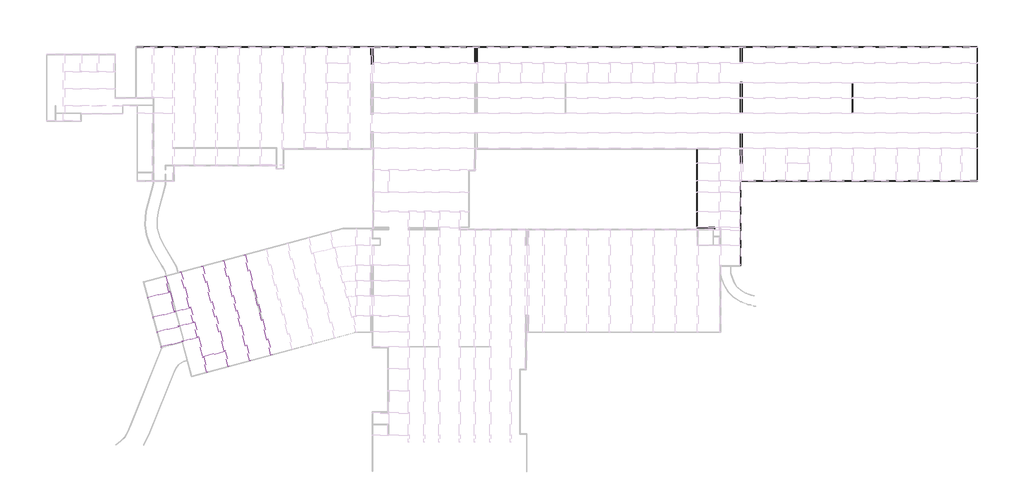
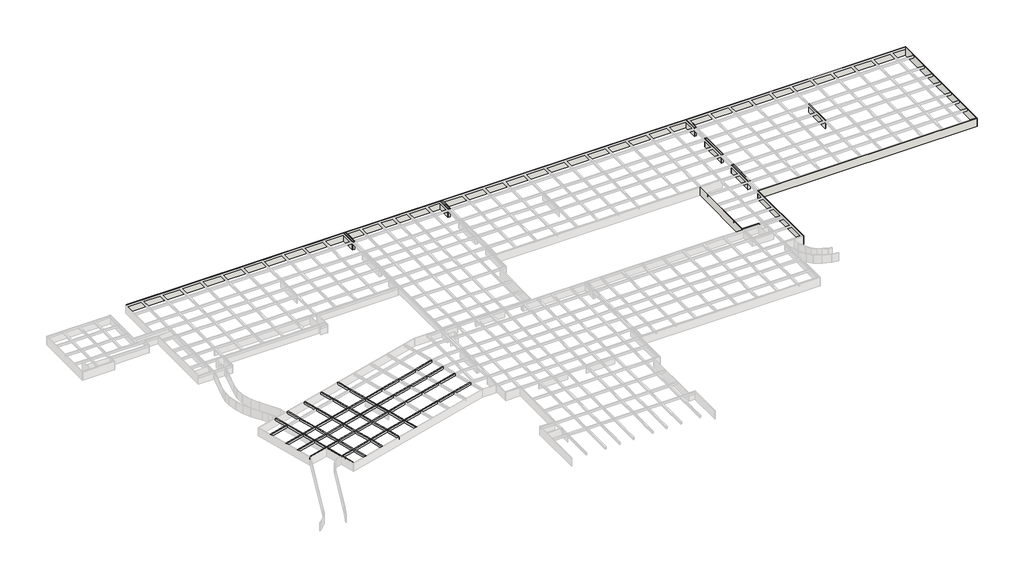
# One storey, part 3 of 14: 25 walls, 10 beams.
"""IFC4 building model written with IfcOpenShell, lengths in millimetres."""

from ifc_helpers import new_model, si_unit, frame, origin, origin_with_axes, place, context, project, spatial, polyline, outline, extrude, faceted_brep, element, save

model = new_model("IFC4")

# Units and contexts
model_context = context("Model", 3, world=origin())
ifc_project = project(units=[si_unit("LENGTHUNIT", "METRE", prefix="MILLI")], contexts=[model_context])

# Site, building, storey
site = spatial("IfcSite", under=ifc_project)
building = spatial("IfcBuilding", under=site)
storey = spatial("IfcBuildingStorey", under=building, Name="户型图", Elevation=0.0)

# Beams
placement = place(None, origin())
element("IfcBeam", 1, ObjectType="混凝土 - 矩形梁 : KL_beam", at=placement, inside=storey, context=model_context, shape_type="Brep", body=[
    faceted_brep([(-44965.652898, -232333.516161, 3300.0), (-45352.02323, -232437.0437735, 3300.0), (-45352.02323, -232437.0437735, 2500.0), (-44965.652898, -232333.516161, 2500.0), (-54495.3696285, -196768.1271004, 3300.0), (-54495.3696285, -196768.1271004, 2500.0), (-54881.7399605, -196871.6547129, 2500.0), (-54881.7399605, -196871.6547129, 3300.0), (-46371.3031308, -227087.5577736, 3300.0), (-46474.8307433, -226701.1874416, 3300.0), (-48238.8947773, -220117.6104614, 3300.0), (-48342.4223897, -219731.2401294, 3300.0), (-49654.0910999, -214836.0255798, 3300.0), (-49757.6187123, -214449.6552478, 3300.0), (-51037.0211351, -209674.8601288, 3300.0), (-51140.5487476, -209288.4897968, 3300.0), (-52926.4464378, -202623.4284974, 3300.0), (-53029.9740503, -202237.0581654, 3300.0), (-53416.344383, -202340.5857754, 3300.0), (-53312.8167705, -202726.9561074, 3300.0), (-51526.9190781, -209392.0174149, 3300.0), (-51423.3914656, -209778.3877469, 3300.0), (-50143.9890429, -214553.1828658, 3300.0), (-50040.4614304, -214939.5531978, 3300.0), (-48728.7927203, -219834.7677475, 3300.0), (-48625.2651078, -220221.1380795, 3300.0), (-46861.2010738, -226804.7150597, 3300.0), (-46757.6734613, -227191.0853917, 3300.0), (-53416.344383, -202340.5857754, 2500.0), (-53312.8167705, -202726.9561074, 2500.0), (-51526.9190781, -209392.0174149, 2500.0), (-51423.3914656, -209778.3877469, 2500.0), (-50143.9890429, -214553.1828658, 2500.0), (-50040.4614304, -214939.5531978, 2500.0), (-48728.7927203, -219834.7677475, 2500.0), (-48625.2651078, -220221.1380795, 2500.0), (-46861.2010738, -226804.7150597, 2500.0), (-46757.6734613, -227191.0853917, 2500.0), (-53029.9740503, -202237.0581654, 2500.0), (-52926.4464378, -202623.4284974, 2500.0), (-51140.5487476, -209288.4897968, 2500.0), (-51037.0211351, -209674.8601288, 2500.0), (-49757.6187123, -214449.6552478, 2500.0), (-49654.0910999, -214836.0255798, 2500.0), (-48342.4223897, -219731.2401294, 2500.0), (-48238.8947773, -220117.6104614, 2500.0), (-46474.8307433, -226701.1874416, 2500.0), (-46371.3031308, -227087.5577736, 2500.0)], [[[0, 1, 2, 3]], [[4, 5, 6, 7]], [[1, 0, 8, 9, 10, 11, 12, 13, 14, 15, 16, 17, 4, 7, 18, 19, 20, 21, 22, 23, 24, 25, 26, 27]], [[2, 1, 27, 26, 25, 24, 23, 22, 21, 20, 19, 18, 7, 6, 28, 29, 30, 31, 32, 33, 34, 35, 36, 37]], [[3, 2, 37, 36, 35, 34, 33, 32, 31, 30, 29, 28, 6, 5, 38, 39, 40, 41, 42, 43, 44, 45, 46, 47]], [[0, 3, 47, 46, 45, 44, 43, 42, 41, 40, 39, 38, 5, 4, 17, 16, 15, 14, 13, 12, 11, 10, 9, 8]]]),
])
element("IfcBeam", 2, ObjectType="混凝土 - 矩形梁 : KL_beam", at=placement, inside=storey, context=model_context, shape_type="Brep", body=[
    faceted_brep([(-47247.810521, -194958.9155951, 3300.0), (-46861.4401905, -194855.3879771, 3300.0), (-46861.4401905, -194855.3879771, 2500.0), (-47247.810521, -194958.9155951, 2500.0), (-37756.1396799, -230382.3134226, 3300.0), (-37756.1396799, -230382.3134226, 2500.0), (-37369.7693494, -230278.7858046, 2500.0), (-37369.7693494, -230278.7858046, 3300.0), (-45815.6063502, -200303.9743273, 3300.0), (-45712.0787322, -200690.3446578, 3300.0), (-43926.1809866, -207355.4057814, 3300.0), (-43822.6533686, -207741.7761119, 3300.0), (-42543.2508773, -212516.5712125, 3300.0), (-42439.7232593, -212902.941543, 3300.0), (-41128.054479, -217798.1560738, 3300.0), (-41024.5268609, -218184.5264043, 3300.0), (-39260.4627326, -224768.1033592, 3300.0), (-39156.9351145, -225154.4736897, 3300.0), (-38770.564784, -225050.9460717, 3300.0), (-38874.092402, -224664.5757412, 3300.0), (-40638.1565304, -218080.9987863, 3300.0), (-40741.6841484, -217694.6284558, 3300.0), (-42053.3529288, -212799.4139249, 3300.0), (-42156.8805468, -212413.0435944, 3300.0), (-43436.283038, -207638.2484938, 3300.0), (-43539.8106561, -207251.8781633, 3300.0), (-45325.7083995, -200586.8170478, 3300.0), (-45429.2360175, -200200.4467173, 3300.0), (-38770.564784, -225050.9460717, 2500.0), (-38874.092402, -224664.5757412, 2500.0), (-40638.1565304, -218080.9987863, 2500.0), (-40741.6841484, -217694.6284558, 2500.0), (-42053.3529288, -212799.4139249, 2500.0), (-42156.8805468, -212413.0435944, 2500.0), (-43436.283038, -207638.2484938, 2500.0), (-43539.8106561, -207251.8781633, 2500.0), (-45325.7083995, -200586.8170478, 2500.0), (-45429.2360175, -200200.4467173, 2500.0), (-39156.9351145, -225154.4736897, 2500.0), (-39260.4627326, -224768.1033592, 2500.0), (-41024.5268609, -218184.5264043, 2500.0), (-41128.054479, -217798.1560738, 2500.0), (-42439.7232593, -212902.941543, 2500.0), (-42543.2508773, -212516.5712125, 2500.0), (-43822.6533686, -207741.7761119, 2500.0), (-43926.1809866, -207355.4057814, 2500.0), (-45712.0787322, -200690.3446578, 2500.0), (-45815.6063502, -200303.9743273, 2500.0)], [[[0, 1, 2, 3]], [[4, 5, 6, 7]], [[1, 0, 8, 9, 10, 11, 12, 13, 14, 15, 16, 17, 4, 7, 18, 19, 20, 21, 22, 23, 24, 25, 26, 27]], [[2, 1, 27, 26, 25, 24, 23, 22, 21, 20, 19, 18, 7, 6, 28, 29, 30, 31, 32, 33, 34, 35, 36, 37]], [[3, 2, 37, 36, 35, 34, 33, 32, 31, 30, 29, 28, 6, 5, 38, 39, 40, 41, 42, 43, 44, 45, 46, 47]], [[0, 3, 47, 46, 45, 44, 43, 42, 41, 40, 39, 38, 5, 4, 17, 16, 15, 14, 13, 12, 11, 10, 9, 8]]]),
])
element("IfcBeam", 3, ObjectType="混凝土 - 矩形梁 : KL_beam", at=placement, inside=storey, context=model_context, shape_type="Brep", body=[
    faceted_brep([(-29827.2079849, -228304.2895391, 3300.0), (-30213.5783169, -228407.8171516, 3300.0), (-30213.5783169, -228407.8171516, 2500.0), (-29827.2079849, -228304.2895391, 2500.0), (-39323.7958794, -192862.5389847, 3300.0), (-39323.7958794, -192862.5389847, 2500.0), (-39710.1662114, -192966.0665972, 2500.0), (-39710.1662114, -192966.0665972, 3300.0), (-31239.6350842, -223033.0395404, 3300.0), (-31343.1626967, -222646.6692084, 3300.0), (-33107.2267306, -216063.0922282, 3300.0), (-33210.7543431, -215676.7218962, 3300.0), (-34522.4230532, -210781.5073465, 3300.0), (-34625.9506657, -210395.1370145, 3300.0), (-35905.3530884, -205620.3418956, 3300.0), (-36008.8807009, -205233.9715636, 3300.0), (-37794.7783067, -198568.9105793, 3300.0), (-37898.3059192, -198182.5402473, 3300.0), (-38284.6762519, -198286.0678573, 3300.0), (-38181.1486394, -198672.4381893, 3300.0), (-36395.2510314, -205337.4991816, 3300.0), (-36291.7234189, -205723.8695136, 3300.0), (-35012.3209962, -210498.6646326, 3300.0), (-34908.7933837, -210885.0349646, 3300.0), (-33597.1246736, -215780.2495142, 3300.0), (-33493.5970611, -216166.6198462, 3300.0), (-31729.5330272, -222750.1968264, 3300.0), (-31626.0054147, -223136.5671584, 3300.0), (-38284.6762519, -198286.0678573, 2500.0), (-38181.1486394, -198672.4381893, 2500.0), (-36395.2510314, -205337.4991816, 2500.0), (-36291.7234189, -205723.8695136, 2500.0), (-35012.3209962, -210498.6646326, 2500.0), (-34908.7933837, -210885.0349646, 2500.0), (-33597.1246736, -215780.2495142, 2500.0), (-33493.5970611, -216166.6198462, 2500.0), (-31729.5330272, -222750.1968264, 2500.0), (-31626.0054147, -223136.5671584, 2500.0), (-37898.3059192, -198182.5402473, 2500.0), (-37794.7783067, -198568.9105793, 2500.0), (-36008.8807009, -205233.9715636, 2500.0), (-35905.3530884, -205620.3418956, 2500.0), (-34625.9506657, -210395.1370145, 2500.0), (-34522.4230532, -210781.5073465, 2500.0), (-33210.7543431, -215676.7218962, 2500.0), (-33107.2267306, -216063.0922282, 2500.0), (-31343.1626967, -222646.6692084, 2500.0), (-31239.6350842, -223033.0395404, 2500.0)], [[[0, 1, 2, 3]], [[4, 5, 6, 7]], [[1, 0, 8, 9, 10, 11, 12, 13, 14, 15, 16, 17, 4, 7, 18, 19, 20, 21, 22, 23, 24, 25, 26, 27]], [[2, 1, 27, 26, 25, 24, 23, 22, 21, 20, 19, 18, 7, 6, 28, 29, 30, 31, 32, 33, 34, 35, 36, 37]], [[3, 2, 37, 36, 35, 34, 33, 32, 31, 30, 29, 28, 6, 5, 38, 39, 40, 41, 42, 43, 44, 45, 46, 47]], [[0, 3, 47, 46, 45, 44, 43, 42, 41, 40, 39, 38, 5, 4, 17, 16, 15, 14, 13, 12, 11, 10, 9, 8]]]),
])
element("IfcBeam", 4, ObjectType="混凝土 - 矩形梁 : KL_beam", at=placement, inside=storey, context=model_context, shape_type="Brep", body=[
    faceted_brep([(-32148.967433, -190913.2453078, 3300.0), (-31762.5971024, -190809.7176898, 3300.0), (-31762.5971024, -190809.7176898, 2500.0), (-32148.967433, -190913.2453078, 2500.0), (-22658.0730491, -226333.7453578, 3300.0), (-22658.0730491, -226333.7453578, 2500.0), (-22271.7027185, -226230.2177398, 2500.0), (-22271.7027185, -226230.2177398, 3300.0), (-30716.7763091, -196258.2553482, 3300.0), (-30613.2486911, -196644.6256787, 3300.0), (-28827.3510298, -203309.6864878, 3300.0), (-28723.8234117, -203696.0568183, 3300.0), (-27444.4209205, -208470.8519189, 3300.0), (-27340.8933025, -208857.2222494, 3300.0), (-26029.2245221, -213752.4367802, 3300.0), (-25925.6969041, -214138.8071108, 3300.0), (-24161.6327757, -220722.3840656, 3300.0), (-24058.1051577, -221108.7543962, 3300.0), (-23671.7348272, -221005.2267781, 3300.0), (-23775.2624452, -220618.8564476, 3300.0), (-25539.3265736, -214035.2794927, 3300.0), (-25642.8541916, -213648.9091622, 3300.0), (-26954.522972, -208753.6946314, 3300.0), (-27058.05059, -208367.3243008, 3300.0), (-28337.4530812, -203592.5292002, 3300.0), (-28440.9806993, -203206.1588697, 3300.0), (-30226.8783584, -196541.0980687, 3300.0), (-30330.4059764, -196154.7277382, 3300.0), (-23671.7348272, -221005.2267781, 2500.0), (-23775.2624452, -220618.8564476, 2500.0), (-25539.3265736, -214035.2794927, 2500.0), (-25642.8541916, -213648.9091622, 2500.0), (-26954.522972, -208753.6946314, 2500.0), (-27058.05059, -208367.3243008, 2500.0), (-28337.4530812, -203592.5292002, 2500.0), (-28440.9806993, -203206.1588697, 2500.0), (-30226.8783584, -196541.0980687, 2500.0), (-30330.4059764, -196154.7277382, 2500.0), (-24058.1051577, -221108.7543962, 2500.0), (-24161.6327757, -220722.3840656, 2500.0), (-25925.6969041, -214138.8071108, 2500.0), (-26029.2245221, -213752.4367802, 2500.0), (-27340.8933025, -208857.2222494, 2500.0), (-27444.4209205, -208470.8519189, 2500.0), (-28723.8234117, -203696.0568183, 2500.0), (-28827.3510298, -203309.6864878, 2500.0), (-30613.2486911, -196644.6256787, 2500.0), (-30716.7763091, -196258.2553482, 2500.0)], [[[0, 1, 2, 3]], [[4, 5, 6, 7]], [[1, 0, 8, 9, 10, 11, 12, 13, 14, 15, 16, 17, 4, 7, 18, 19, 20, 21, 22, 23, 24, 25, 26, 27]], [[2, 1, 27, 26, 25, 24, 23, 22, 21, 20, 19, 18, 7, 6, 28, 29, 30, 31, 32, 33, 34, 35, 36, 37]], [[3, 2, 37, 36, 35, 34, 33, 32, 31, 30, 29, 28, 6, 5, 38, 39, 40, 41, 42, 43, 44, 45, 46, 47]], [[0, 3, 47, 46, 45, 44, 43, 42, 41, 40, 39, 38, 5, 4, 17, 16, 15, 14, 13, 12, 11, 10, 9, 8]]]),
])
element("IfcBeam", 5, ObjectType="混凝土 - 矩形梁 : KL_beam", at=placement, inside=storey, context=model_context, shape_type="SweptSolid", body=[
    extrude(outline(polyline([(-66208.1826107, -206224.0134222), (-66313.6007329, -205838.1546145), (-58837.3326561, -203795.609192), (-58733.7322459, -204181.9646057), (-66208.1826107, -206224.0134222)])), frame((0.0, 0.0, 2500.0), z_axis=(0.0, 0.0, 1.0), x_axis=(1.0, 0.0, 0.0)), (0.0, 0.0, 1.0), 800.0),
])
element("IfcBeam", 6, ObjectType="混凝土 - 矩形梁 : KL_beam", at=placement, inside=storey, context=model_context, shape_type="Brep", body=[
    faceted_brep([(-64399.4506069, -212841.2018425, 3300.0), (-64399.4506069, -212841.2018425, 2500.0), (-64295.9229889, -213227.5721731, 2500.0), (-64295.9229889, -213227.5721731, 3300.0), (-51526.9190781, -209392.0174149, 3300.0), (-51423.3914656, -209778.3877469, 3300.0), (-51423.3914656, -209778.3877469, 2500.0), (-51526.9190781, -209392.0174149, 2500.0), (-56843.6193706, -211230.7334368, 3300.0), (-56457.2490334, -211127.205817, 3300.0), (-56560.8482958, -210740.8546835, 3300.0), (-56947.218633, -210844.3823033, 3300.0), (-56843.6193706, -211230.7334368, 2500.0), (-56457.2490334, -211127.205817, 2500.0), (-56947.218633, -210844.3823033, 2500.0), (-56560.8482958, -210740.8546835, 2500.0)], [[[0, 1, 2, 3]], [[4, 5, 6, 7]], [[0, 3, 8, 9, 5, 4, 10, 11]], [[3, 2, 12, 13, 6, 5, 9, 8]], [[2, 1, 14, 15, 7, 6, 13, 12]], [[1, 0, 11, 10, 4, 7, 15, 14]]]),
    faceted_brep([(-51140.5487476, -209288.4897968, 3300.0), (-51037.0211351, -209674.8601288, 3300.0), (-43822.6533686, -207741.7761119, 3300.0), (-43926.1809866, -207355.4057814, 3300.0), (-51037.0211351, -209674.8601288, 2500.0), (-43822.6533686, -207741.7761119, 2500.0), (-51140.5487476, -209288.4897968, 2500.0), (-43926.1809866, -207355.4057814, 2500.0)], [[[0, 1, 2, 3]], [[1, 4, 5, 2]], [[4, 6, 7, 5]], [[6, 0, 3, 7]], [[1, 0, 6, 4]], [[3, 2, 5, 7]]]),
    faceted_brep([(1279.8377522, -195242.4895673, 3300.0), (1383.3653703, -195628.8598978, 3300.0), (1383.3653703, -195628.8598978, 2500.0), (1279.8377522, -195242.4895673, 2500.0), (-5935.794677, -197175.9124495, 3300.0), (-5832.1954146, -197562.263583, 3300.0), (-5832.1954146, -197562.263583, 2500.0), (-5935.794677, -197175.9124495, 2500.0)], [[[0, 1, 2, 3]], [[1, 0, 4, 5]], [[2, 1, 5, 6]], [[3, 2, 6, 7]], [[0, 3, 7, 4]], [[5, 4, 7, 6]]]),
    faceted_brep([(-43436.283038, -207638.2484938, 3300.0), (-43539.8106561, -207251.8781633, 3300.0), (-43539.8106561, -207251.8781633, 2500.0), (-43436.283038, -207638.2484938, 2500.0), (-36395.2510314, -205337.4991816, 3300.0), (-36291.7234189, -205723.8695136, 3300.0), (-36291.7234189, -205723.8695136, 2500.0), (-36395.2510314, -205337.4991816, 2500.0)], [[[0, 1, 2, 3]], [[4, 5, 6, 7]], [[1, 0, 5, 4]], [[0, 3, 6, 5]], [[3, 2, 7, 6]], [[2, 1, 4, 7]]]),
    faceted_brep([(-36008.8807009, -205233.9715636, 3300.0), (-35905.3530884, -205620.3418956, 3300.0), (-28723.8234117, -203696.0568183, 3300.0), (-28827.3510298, -203309.6864878, 3300.0), (-35905.3530884, -205620.3418956, 2500.0), (-28723.8234117, -203696.0568183, 2500.0), (-36008.8807009, -205233.9715636, 2500.0), (-28827.3510298, -203309.6864878, 2500.0)], [[[0, 1, 2, 3]], [[1, 4, 5, 2]], [[4, 6, 7, 5]], [[6, 0, 3, 7]], [[1, 0, 6, 4]], [[3, 2, 5, 7]]]),
    faceted_brep([(-28337.4530812, -203592.5292002, 3300.0), (-28440.9806993, -203206.1588697, 3300.0), (-28440.9806993, -203206.1588697, 2500.0), (-28337.4530812, -203592.5292002, 2500.0), (-21391.9678165, -201317.3815604, 3300.0), (-21288.3685541, -201703.7326938, 3300.0), (-21288.3685541, -201703.7326938, 2500.0), (-21391.9678165, -201317.3815604, 2500.0)], [[[0, 1, 2, 3]], [[4, 5, 6, 7]], [[1, 0, 5, 4]], [[0, 3, 6, 5]], [[3, 2, 7, 6]], [[2, 1, 4, 7]]]),
    faceted_brep([(-21005.5974794, -201213.8539405, 3300.0), (-20901.9982169, -201600.205074, 3300.0), (-13710.1170819, -199673.1463318, 3300.0), (-13813.6447, -199286.7760013, 3300.0), (-20901.9982169, -201600.205074, 2500.0), (-13710.1170819, -199673.1463318, 2500.0), (-21005.5974794, -201213.8539405, 2500.0), (-13813.6447, -199286.7760013, 2500.0)], [[[0, 1, 2, 3]], [[1, 4, 5, 2]], [[4, 6, 7, 5]], [[6, 0, 3, 7]], [[1, 0, 6, 4]], [[3, 2, 5, 7]]]),
    faceted_brep([(-13323.7467514, -199569.6187138, 3300.0), (-13427.2743694, -199183.2483833, 3300.0), (-13427.2743694, -199183.2483833, 2500.0), (-13323.7467514, -199569.6187138, 2500.0), (-6322.1650141, -197279.4400694, 3300.0), (-6218.5657517, -197665.7912028, 3300.0), (-6218.5657517, -197665.7912028, 2500.0), (-6322.1650141, -197279.4400694, 2500.0)], [[[0, 1, 2, 3]], [[4, 5, 6, 7]], [[1, 0, 5, 4]], [[0, 3, 6, 5]], [[3, 2, 7, 6]], [[2, 1, 4, 7]]]),
])
element("IfcBeam", 7, ObjectType="混凝土 - 矩形梁 : KL_beam", at=placement, inside=storey, context=model_context, shape_type="Brep", body=[
    faceted_brep([(-62991.3282704, -217995.6170367, 3300.0), (-62991.3282704, -217995.6170367, 2500.0), (-62887.8006524, -218381.9873672, 2500.0), (-62887.8006524, -218381.9873672, 3300.0), (-50143.9890429, -214553.1828658, 3300.0), (-50040.4614304, -214939.5531978, 3300.0), (-50040.4614304, -214939.5531978, 2500.0), (-50143.9890429, -214553.1828658, 2500.0), (-55459.7322302, -216391.6424322, 3300.0), (-55073.361893, -216288.1148124, 3300.0), (-55176.9611554, -215901.7636789, 3300.0), (-55563.3314926, -216005.2912987, 3300.0), (-55459.7322302, -216391.6424322, 2500.0), (-55073.361893, -216288.1148124, 2500.0), (-55563.3314926, -216005.2912987, 2500.0), (-55176.9611554, -215901.7636789, 2500.0)], [[[0, 1, 2, 3]], [[4, 5, 6, 7]], [[0, 3, 8, 9, 5, 4, 10, 11]], [[3, 2, 12, 13, 6, 5, 9, 8]], [[2, 1, 14, 15, 7, 6, 13, 12]], [[1, 0, 11, 10, 4, 7, 15, 14]]]),
    faceted_brep([(-49757.6187123, -214449.6552478, 3300.0), (-49654.0910999, -214836.0255798, 3300.0), (-42439.7232593, -212902.941543, 3300.0), (-42543.2508773, -212516.5712125, 3300.0), (-49654.0910999, -214836.0255798, 2500.0), (-42439.7232593, -212902.941543, 2500.0), (-49757.6187123, -214449.6552478, 2500.0), (-42543.2508773, -212516.5712125, 2500.0)], [[[0, 1, 2, 3]], [[1, 4, 5, 2]], [[4, 6, 7, 5]], [[6, 0, 3, 7]], [[1, 0, 6, 4]], [[3, 2, 5, 7]]]),
    faceted_brep([(2662.7678615, -200403.6549984, 3300.0), (2766.2954795, -200790.0253289, 3300.0), (2766.2954795, -200790.0253289, 2500.0), (2662.7678615, -200403.6549984, 2500.0), (-4551.9075366, -202336.8214449, 3300.0), (-4448.3082742, -202723.1725784, 3300.0), (-4448.3082742, -202723.1725784, 2500.0), (-4551.9075366, -202336.8214449, 2500.0)], [[[0, 1, 2, 3]], [[1, 0, 4, 5]], [[2, 1, 5, 6]], [[3, 2, 6, 7]], [[0, 3, 7, 4]], [[5, 4, 7, 6]]]),
    faceted_brep([(-42053.3529288, -212799.4139249, 3300.0), (-42156.8805468, -212413.0435944, 3300.0), (-42156.8805468, -212413.0435944, 2500.0), (-42053.3529288, -212799.4139249, 2500.0), (-35012.3209962, -210498.6646326, 3300.0), (-34908.7933837, -210885.0349646, 3300.0), (-34908.7933837, -210885.0349646, 2500.0), (-35012.3209962, -210498.6646326, 2500.0)], [[[0, 1, 2, 3]], [[4, 5, 6, 7]], [[1, 0, 5, 4]], [[0, 3, 6, 5]], [[3, 2, 7, 6]], [[2, 1, 4, 7]]]),
    faceted_brep([(-34625.9506657, -210395.1370145, 3300.0), (-34522.4230532, -210781.5073465, 3300.0), (-27340.8933025, -208857.2222494, 3300.0), (-27444.4209205, -208470.8519189, 3300.0), (-34522.4230532, -210781.5073465, 2500.0), (-27340.8933025, -208857.2222494, 2500.0), (-34625.9506657, -210395.1370145, 2500.0), (-27444.4209205, -208470.8519189, 2500.0)], [[[0, 1, 2, 3]], [[1, 4, 5, 2]], [[4, 6, 7, 5]], [[6, 0, 3, 7]], [[1, 0, 6, 4]], [[3, 2, 5, 7]]]),
    faceted_brep([(-26954.522972, -208753.6946314, 3300.0), (-27058.05059, -208367.3243008, 3300.0), (-27058.05059, -208367.3243008, 2500.0), (-26954.522972, -208753.6946314, 2500.0), (-20008.0806761, -206478.2905558, 3300.0), (-19904.4814137, -206864.6416892, 3300.0), (-19904.4814137, -206864.6416892, 2500.0), (-20008.0806761, -206478.2905558, 2500.0)], [[[0, 1, 2, 3]], [[4, 5, 6, 7]], [[1, 0, 5, 4]], [[0, 3, 6, 5]], [[3, 2, 7, 6]], [[2, 1, 4, 7]]]),
    faceted_brep([(-19621.710339, -206374.7629359, 3300.0), (-19518.1110766, -206761.1140694, 3300.0), (-12327.1869726, -204834.3117629, 3300.0), (-12430.7145907, -204447.9414324, 3300.0), (-19518.1110766, -206761.1140694, 2500.0), (-12327.1869726, -204834.3117629, 2500.0), (-19621.710339, -206374.7629359, 2500.0), (-12430.7145907, -204447.9414324, 2500.0)], [[[0, 1, 2, 3]], [[1, 4, 5, 2]], [[4, 6, 7, 5]], [[6, 0, 3, 7]], [[1, 0, 6, 4]], [[3, 2, 5, 7]]]),
    faceted_brep([(-11940.8166421, -204730.7841449, 3300.0), (-12044.3442602, -204344.4138144, 3300.0), (-12044.3442602, -204344.4138144, 2500.0), (-11940.8166421, -204730.7841449, 2500.0), (-4938.2778738, -202440.3490648, 3300.0), (-4834.6786113, -202826.7001982, 3300.0), (-4834.6786113, -202826.7001982, 2500.0), (-4938.2778738, -202440.3490648, 2500.0)], [[[0, 1, 2, 3]], [[4, 5, 6, 7]], [[1, 0, 5, 4]], [[0, 3, 6, 5]], [[3, 2, 7, 6]], [[2, 1, 4, 7]]]),
])
element("IfcBeam", 8, ObjectType="混凝土 - 矩形梁 : KL_beam", at=placement, inside=storey, context=model_context, shape_type="Brep", body=[
    faceted_brep([(-61550.1618798, -223270.2432596, 3300.0), (-61550.1618798, -223270.2432596, 2500.0), (-61446.6342617, -223656.6135901, 2500.0), (-61446.6342617, -223656.6135901, 3300.0), (-48728.7927203, -219834.7677475, 3300.0), (-48625.2651078, -220221.1380795, 3300.0), (-48625.2651078, -220221.1380795, 2500.0), (-48728.7927203, -219834.7677475, 2500.0), (-54043.5564714, -221672.9648747, 3300.0), (-53657.1861343, -221569.4372549, 3300.0), (-53760.7853967, -221183.0861214, 3300.0), (-54147.1557338, -221286.6137413, 3300.0), (-54043.5564714, -221672.9648747, 2500.0), (-53657.1861343, -221569.4372549, 2500.0), (-54147.1557338, -221286.6137413, 2500.0), (-53760.7853967, -221183.0861214, 2500.0)], [[[0, 1, 2, 3]], [[4, 5, 6, 7]], [[0, 3, 8, 9, 5, 4, 10, 11]], [[3, 2, 12, 13, 6, 5, 9, 8]], [[2, 1, 14, 15, 7, 6, 13, 12]], [[1, 0, 11, 10, 4, 7, 15, 14]]]),
    faceted_brep([(-48342.4223897, -219731.2401294, 3300.0), (-48238.8947773, -220117.6104614, 3300.0), (-41024.5268609, -218184.5264043, 3300.0), (-41128.054479, -217798.1560738, 3300.0), (-48238.8947773, -220117.6104614, 2500.0), (-41024.5268609, -218184.5264043, 2500.0), (-48342.4223897, -219731.2401294, 2500.0), (-41128.054479, -217798.1560738, 2500.0)], [[[0, 1, 2, 3]], [[1, 4, 5, 2]], [[4, 6, 7, 5]], [[6, 0, 3, 7]], [[1, 0, 6, 4]], [[3, 2, 5, 7]]]),
    faceted_brep([(4077.9642599, -205685.2398597, 3300.0), (4181.4918779, -206071.6101903, 3300.0), (4181.4918779, -206071.6101903, 2500.0), (4077.9642599, -205685.2398597, 2500.0), (-3135.7317778, -207618.1438875, 3300.0), (-3032.1325154, -208004.4950209, 3300.0), (-3032.1325154, -208004.4950209, 2500.0), (-3135.7317778, -207618.1438875, 2500.0)], [[[0, 1, 2, 3]], [[1, 0, 4, 5]], [[2, 1, 5, 6]], [[3, 2, 6, 7]], [[0, 3, 7, 4]], [[5, 4, 7, 6]]]),
    faceted_brep([(-40638.1565304, -218080.9987863, 3300.0), (-40741.6841484, -217694.6284558, 3300.0), (-40741.6841484, -217694.6284558, 2500.0), (-40638.1565304, -218080.9987863, 2500.0), (-33597.1246736, -215780.2495142, 3300.0), (-33493.5970611, -216166.6198462, 3300.0), (-33493.5970611, -216166.6198462, 2500.0), (-33597.1246736, -215780.2495142, 2500.0)], [[[0, 1, 2, 3]], [[4, 5, 6, 7]], [[1, 0, 5, 4]], [[0, 3, 6, 5]], [[3, 2, 7, 6]], [[2, 1, 4, 7]]]),
    faceted_brep([(-33210.7543431, -215676.7218962, 3300.0), (-33107.2267306, -216063.0922282, 3300.0), (-25925.6969041, -214138.8071108, 3300.0), (-26029.2245221, -213752.4367802, 3300.0), (-33107.2267306, -216063.0922282, 2500.0), (-25925.6969041, -214138.8071108, 2500.0), (-33210.7543431, -215676.7218962, 2500.0), (-26029.2245221, -213752.4367802, 2500.0)], [[[0, 1, 2, 3]], [[1, 4, 5, 2]], [[4, 6, 7, 5]], [[6, 0, 3, 7]], [[1, 0, 6, 4]], [[3, 2, 5, 7]]]),
    faceted_brep([(-25539.3265736, -214035.2794927, 3300.0), (-25642.8541916, -213648.9091622, 3300.0), (-25642.8541916, -213648.9091622, 2500.0), (-25539.3265736, -214035.2794927, 2500.0), (-18591.9049174, -211759.6129983, 3300.0), (-18488.305655, -212145.9641318, 3300.0), (-18488.305655, -212145.9641318, 2500.0), (-18591.9049174, -211759.6129983, 2500.0)], [[[0, 1, 2, 3]], [[4, 5, 6, 7]], [[1, 0, 5, 4]], [[0, 3, 6, 5]], [[3, 2, 7, 6]], [[2, 1, 4, 7]]]),
    faceted_brep([(-18205.5345802, -211656.0853785, 3300.0), (-18101.9353178, -212042.4365119, 3300.0), (-10911.9905743, -210115.8966243, 3300.0), (-11015.5181923, -209729.5262938, 3300.0), (-18101.9353178, -212042.4365119, 2500.0), (-10911.9905743, -210115.8966243, 2500.0), (-18205.5345802, -211656.0853785, 2500.0), (-11015.5181923, -209729.5262938, 2500.0)], [[[0, 1, 2, 3]], [[1, 4, 5, 2]], [[4, 6, 7, 5]], [[6, 0, 3, 7]], [[1, 0, 6, 4]], [[3, 2, 5, 7]]]),
    faceted_brep([(-10525.6202438, -210012.3690062, 3300.0), (-10629.1478618, -209625.9986757, 3300.0), (-10629.1478618, -209625.9986757, 2500.0), (-10525.6202438, -210012.3690062, 2500.0), (-3522.102115, -207721.6715073, 3300.0), (-3418.5028526, -208108.0226408, 3300.0), (-3418.5028526, -208108.0226408, 2500.0), (-3522.102115, -207721.6715073, 2500.0)], [[[0, 1, 2, 3]], [[4, 5, 6, 7]], [[1, 0, 5, 4]], [[0, 3, 6, 5]], [[3, 2, 7, 6]], [[2, 1, 4, 7]]]),
])
element("IfcBeam", 9, ObjectType="混凝土 - 矩形梁 : KL_beam", at=placement, inside=storey, context=model_context, shape_type="SweptSolid", body=[
    extrude(outline(polyline([(5945.5560063, -212655.1871451), (6049.0836243, -213041.5574756), (-1163.2483368, -214974.0960002), (-1266.8475992, -214587.7448667), (5945.5560063, -212655.1871451)])), frame((0.0, 0.0, 2500.0), z_axis=(0.0, 0.0, 1.0), x_axis=(1.0, 0.0, 0.0)), (0.0, 0.0, 1.0), 800.0),
    extrude(outline(polyline([(-46861.2010738, -226804.7150597), (-46757.6734613, -227191.0853917), (-51788.3019556, -228539.0382341), (-51891.9012181, -228152.6871007), (-46861.2010738, -226804.7150597)])), frame((0.0, 0.0, 2500.0), z_axis=(0.0, 0.0, 1.0), x_axis=(1.0, 0.0, 0.0)), (0.0, 0.0, 1.0), 800.0),
    extrude(outline(polyline([(-46371.3031308, -227087.5577736), (-46474.8307433, -226701.1874416), (-39260.4627326, -224768.1033592), (-39156.9351145, -225154.4736897), (-46371.3031308, -227087.5577736)])), frame((0.0, 0.0, 2500.0), z_axis=(0.0, 0.0, 1.0), x_axis=(1.0, 0.0, 0.0)), (0.0, 0.0, 1.0), 800.0),
    extrude(outline(polyline([(-31626.0054147, -223136.5671584), (-38770.564784, -225050.9460717), (-38874.092402, -224664.5757412), (-31729.5330272, -222750.1968264), (-31626.0054147, -223136.5671584)])), frame((0.0, 0.0, 2500.0), z_axis=(0.0, 0.0, 1.0), x_axis=(1.0, 0.0, 0.0)), (0.0, 0.0, 1.0), 800.0),
    extrude(outline(polyline([(-24058.1051577, -221108.7543962), (-31239.6350842, -223033.0395404), (-31343.1626967, -222646.6692084), (-24161.6327757, -220722.3840656), (-24058.1051577, -221108.7543962)])), frame((0.0, 0.0, 2500.0), z_axis=(0.0, 0.0, 1.0), x_axis=(1.0, 0.0, 0.0)), (0.0, 0.0, 1.0), 800.0),
    extrude(outline(polyline([(-16619.4214764, -219115.565111), (-23671.7348272, -221005.2267781), (-23775.2624452, -220618.8564476), (-16723.0207388, -218729.2139775), (-16619.4214764, -219115.565111)])), frame((0.0, 0.0, 2500.0), z_axis=(0.0, 0.0, 1.0), x_axis=(1.0, 0.0, 0.0)), (0.0, 0.0, 1.0), 800.0),
    extrude(outline(polyline([(-9044.3988279, -217085.8439097), (-16233.0511392, -219012.0374912), (-16336.6504016, -218625.6863577), (-9147.9264459, -216699.4735792), (-9044.3988279, -217085.8439097)])), frame((0.0, 0.0, 2500.0), z_axis=(0.0, 0.0, 1.0), x_axis=(1.0, 0.0, 0.0)), (0.0, 0.0, 1.0), 800.0),
    extrude(outline(polyline([(-1549.618674, -215077.62362), (-8658.0284974, -216982.3162916), (-8761.5561154, -216595.9459611), (-1653.2179364, -214691.2724865), (-1549.618674, -215077.62362)])), frame((0.0, 0.0, 2500.0), z_axis=(0.0, 0.0, 1.0), x_axis=(1.0, 0.0, 0.0)), (0.0, 0.0, 1.0), 800.0),
])
element("IfcBeam", 10, ObjectType="混凝土 - 矩形梁 : KL_beam", at=placement, inside=storey, context=model_context, shape_type="Brep", body=[
    faceted_brep([(-50406.0295376, -233693.9254706, 3300.0), (-50792.3806644, -233797.5247312, 3300.0), (-50792.3806644, -233797.5247312, 2500.0), (-50406.0295376, -233693.9254706, 2500.0), (-51788.3019556, -228539.0382341, 3300.0), (-51891.9012181, -228152.6871007, 3300.0), (-53657.1861343, -221569.4372549, 3300.0), (-54043.5564714, -221672.9648747, 3300.0), (-54043.5564714, -221672.9648747, 2500.0), (-53657.1861343, -221569.4372549, 2500.0), (-51891.9012181, -228152.6871007, 2500.0), (-51788.3019556, -228539.0382341, 2500.0)], [[[0, 1, 2, 3]], [[1, 0, 4, 5, 6, 7]], [[2, 1, 7, 8]], [[3, 2, 8, 9, 10, 11]], [[0, 3, 11, 10, 9, 6, 5, 4]], [[7, 6, 9, 8]]]),
    faceted_brep([(-59881.2179144, -198358.2514113, 3300.0), (-59881.2179144, -198358.2514113, 2500.0), (-60267.5690413, -198461.8506719, 2500.0), (-60267.5690413, -198461.8506719, 3300.0), (-56560.8482958, -210740.8546835, 3300.0), (-56947.218633, -210844.3823033, 3300.0), (-56947.218633, -210844.3823033, 2500.0), (-56560.8482958, -210740.8546835, 2500.0), (-58837.3326561, -203795.609192, 3300.0), (-58733.7322459, -204181.9646057, 3300.0), (-58347.9820093, -204076.1244544, 3300.0), (-58451.5812717, -203689.773321, 3300.0), (-58837.3326561, -203795.609192, 2500.0), (-58733.7322459, -204181.9646057, 2500.0), (-58451.5812717, -203689.773321, 2500.0), (-58347.9820093, -204076.1244544, 2500.0)], [[[0, 1, 2, 3]], [[4, 5, 6, 7]], [[0, 3, 8, 9, 5, 4, 10, 11]], [[3, 2, 12, 13, 6, 5, 9, 8]], [[2, 1, 14, 15, 7, 6, 13, 12]], [[1, 0, 11, 10, 4, 7, 15, 14]]]),
    faceted_brep([(-56843.6193706, -211230.7334368, 3300.0), (-56457.2490334, -211127.205817, 3300.0), (-56457.2490334, -211127.205817, 2500.0), (-56843.6193706, -211230.7334368, 2500.0), (-55176.9611554, -215901.7636789, 3300.0), (-55563.3314926, -216005.2912987, 3300.0), (-55563.3314926, -216005.2912987, 2500.0), (-55176.9611554, -215901.7636789, 2500.0)], [[[0, 1, 2, 3]], [[4, 5, 6, 7]], [[1, 0, 5, 4]], [[0, 3, 6, 5]], [[3, 2, 7, 6]], [[2, 1, 4, 7]]]),
    faceted_brep([(-55459.7322302, -216391.6424322, 3300.0), (-55073.361893, -216288.1148124, 3300.0), (-55073.361893, -216288.1148124, 2500.0), (-55459.7322302, -216391.6424322, 2500.0), (-53760.7853967, -221183.0861214, 3300.0), (-54147.1557338, -221286.6137413, 3300.0), (-54147.1557338, -221286.6137413, 2500.0), (-53760.7853967, -221183.0861214, 2500.0)], [[[0, 1, 2, 3]], [[4, 5, 6, 7]], [[1, 0, 5, 4]], [[0, 3, 6, 5]], [[3, 2, 7, 6]], [[2, 1, 4, 7]]]),
])

# Walls
element("IfcWall", 11, ObjectType="所有墙体", at=placement, inside=storey, context=model_context, shape_type="Brep", body=[
    faceted_brep([(-70312.7050956, -117418.950757, 0.0), (12717.2949044, -117418.950757, 0.0), (12837.2949044, -117418.950757, 0.0), (13417.2949044, -117418.950757, 0.0), (13537.2949044, -117418.950757, 0.0), (49516.5330009, -117418.950757, 0.0), (49636.5330009, -117418.950757, 0.0), (50217.2949044, -117418.950757, 0.0), (50337.2949044, -117418.950757, 0.0), (143317.2949044, -117418.950757, 0.0), (143437.2949044, -117418.950757, 0.0), (144017.2949044, -117418.950757, 0.0), (144137.2949044, -117418.950757, 0.0), (227167.2949044, -117418.950757, 0.0), (227287.2949044, -117418.950757, 0.0), (227287.2949044, -117418.950757, 3300.0), (227167.2949044, -117418.950757, 3300.0), (144137.2949044, -117418.950757, 3300.0), (144017.2949044, -117418.950757, 3300.0), (143437.2949044, -117418.950757, 3300.0), (143317.2949044, -117418.950757, 3300.0), (50337.2949044, -117418.950757, 3300.0), (50217.2949044, -117418.950757, 3300.0), (49636.5330009, -117418.950757, 3300.0), (49516.5330009, -117418.950757, 3300.0), (13537.2949044, -117418.950757, 3300.0), (13417.2949044, -117418.950757, 3300.0), (12837.2949044, -117418.950757, 3300.0), (12717.2949044, -117418.950757, 3300.0), (-70312.7050956, -117418.950757, 3300.0), (-70312.7050956, -117298.950757, 0.0), (-70312.7050956, -117298.950757, 3300.0), (227287.2949044, -117298.950757, 3300.0), (227287.2949044, -117298.950757, 0.0)], [[[0, 1, 2, 3, 4, 5, 6, 7, 8, 9, 10, 11, 12, 13, 14, 15, 16, 17, 18, 19, 20, 21, 22, 23, 24, 25, 26, 27, 28, 29]], [[30, 31, 32, 33]], [[14, 13, 12, 11, 10, 9, 8, 7, 6, 5, 4, 3, 2, 1, 0, 30, 33]], [[29, 28, 27, 26, 25, 24, 23, 22, 21, 20, 19, 18, 17, 16, 15, 32, 31]], [[0, 29, 31, 30]], [[15, 14, 33, 32]]]),
])
element("IfcWall", 12, ObjectType="所有墙体", at=placement, inside=storey, context=model_context, shape_type="Brep", body=[
    faceted_brep([(227167.2949044, -117418.950757, 0.0), (227167.2949044, -164696.0449275, 0.0), (227167.2949044, -164816.0449275, 0.0), (227167.2949044, -164816.0449275, 3300.0), (227167.2949044, -164696.0449275, 3300.0), (227167.2949044, -117418.950757, 3300.0), (227287.2949044, -117418.950757, 0.0), (227287.2949044, -117418.950757, 3300.0), (227287.2949044, -164816.0449275, 3300.0), (227287.2949044, -164816.0449275, 0.0)], [[[0, 1, 2, 3, 4, 5]], [[6, 7, 8, 9]], [[2, 1, 0, 6, 9]], [[5, 4, 3, 8, 7]], [[0, 5, 7, 6]], [[3, 2, 9, 8]]]),
])
element("IfcWall", 13, ObjectType="所有墙体", at=placement, inside=storey, context=model_context, shape_type="Brep", body=[
    faceted_brep([(227167.2949044, -164696.0449275, 0.0), (143467.2949044, -164696.0449275, 0.0), (143467.2949044, -164696.0449275, 3300.0), (227167.2949044, -164696.0449275, 3300.0), (227167.2949044, -164816.0449275, 0.0), (227167.2949044, -164816.0449275, 3300.0), (143587.2949044, -164816.0449275, 3300.0), (143467.2949044, -164816.0449275, 3300.0), (143467.2949044, -164816.0449275, 0.0), (143587.2949044, -164816.0449275, 0.0)], [[[0, 1, 2, 3]], [[4, 5, 6, 7, 8, 9]], [[1, 0, 4, 9, 8]], [[3, 2, 7, 6, 5]], [[0, 3, 5, 4]], [[2, 1, 8, 7]]]),
])
element("IfcWall", 14, ObjectType="所有墙体", at=placement, inside=storey, context=model_context, shape_type="Brep", body=[
    faceted_brep([(143467.2949044, -164816.0449275, 0.0), (143467.2949044, -194796.0449275, 0.0), (143467.2949044, -194916.0449275, 0.0), (143467.2949044, -194916.0449275, 3300.0), (143467.2949044, -194796.0449275, 3300.0), (143467.2949044, -164816.0449275, 3300.0), (143587.2949044, -164816.0449275, 0.0), (143587.2949044, -164816.0449275, 3300.0), (143587.2949044, -194916.0449275, 3300.0), (143587.2949044, -194916.0449275, 0.0)], [[[0, 1, 2, 3, 4, 5]], [[6, 7, 8, 9]], [[2, 1, 0, 6, 9]], [[5, 4, 3, 8, 7]], [[0, 5, 7, 6]], [[3, 2, 9, 8]]]),
])
element("IfcWall", 15, ObjectType="所有墙体", at=placement, inside=storey, context=model_context, shape_type="Brep", body=[
    faceted_brep([(134428.3552546, -181848.950757, 0.0), (134428.3552546, -181148.950757, 0.0), (134428.3552546, -181148.950757, 3300.0), (134428.3552546, -181848.950757, 3300.0), (134308.3552546, -181848.950757, 0.0), (134308.3552546, -181848.950757, 3300.0), (134308.3552546, -181268.950757, 3300.0), (134308.3552546, -181148.950757, 3300.0), (134308.3552546, -181148.950757, 0.0), (134308.3552546, -181268.950757, 0.0)], [[[0, 1, 2, 3]], [[4, 5, 6, 7, 8, 9]], [[1, 0, 4, 9, 8]], [[3, 2, 7, 6, 5]], [[0, 3, 5, 4]], [[2, 1, 8, 7]]]),
])
element("IfcWall", 16, ObjectType="所有墙体", at=placement, inside=storey, context=model_context, shape_type="Brep", body=[
    faceted_brep([(134308.3552546, -181148.950757, 0.0), (128087.2949044, -181148.950757, 0.0), (127967.2949044, -181148.950757, 0.0), (127967.2949044, -181148.950757, 3300.0), (128087.2949044, -181148.950757, 3300.0), (134308.3552546, -181148.950757, 3300.0), (134308.3552546, -181268.950757, 0.0), (134308.3552546, -181268.950757, 3300.0), (127967.2949044, -181268.950757, 3300.0), (127967.2949044, -181268.950757, 0.0)], [[[0, 1, 2, 3, 4, 5]], [[6, 7, 8, 9]], [[2, 1, 0, 6, 9]], [[5, 4, 3, 8, 7]], [[0, 5, 7, 6]], [[3, 2, 9, 8]]]),
])
element("IfcWall", 17, ObjectType="所有墙体", at=placement, inside=storey, context=model_context, shape_type="SweptSolid", body=[
    extrude(outline(polyline([(128087.2949044, -153418.950757), (128087.2949044, -181148.950757), (127967.2949044, -181148.950757), (127967.2949044, -153418.950757), (128087.2949044, -153418.950757)])), origin_with_axes(), (0.0, 0.0, 1.0), 3300.0),
])
element("IfcWall", 18, ObjectType="所有墙体", at=placement, inside=storey, context=model_context, shape_type="Brep", body=[
    faceted_brep([(143317.2949044, -158518.950757, 0.0), (144137.2949044, -158518.950757, 0.0), (144137.2949044, -158518.950757, 3300.0), (143317.2949044, -158518.950757, 3300.0), (143317.2949044, -158398.950757, 0.0), (143317.2949044, -158398.950757, 3300.0), (143437.2949044, -158398.950757, 3300.0), (144017.2949044, -158398.950757, 3300.0), (144137.2949044, -158398.950757, 3300.0), (144137.2949044, -158398.950757, 0.0), (144017.2949044, -158398.950757, 0.0), (143437.2949044, -158398.950757, 0.0)], [[[0, 1, 2, 3]], [[4, 5, 6, 7, 8, 9, 10, 11]], [[1, 0, 4, 11, 10, 9]], [[3, 2, 8, 7, 6, 5]], [[2, 1, 9, 8]], [[0, 3, 5, 4]]]),
])
element("IfcWall", 19, ObjectType="所有墙体", at=placement, inside=storey, context=model_context, shape_type="Brep", body=[
    faceted_brep([(144137.2949044, -158398.950757, 0.0), (144137.2949044, -147598.950757, 0.0), (144137.2949044, -147598.950757, 3300.0), (144137.2949044, -158398.950757, 3300.0), (144017.2949044, -158398.950757, 0.0), (144017.2949044, -158398.950757, 3300.0), (144017.2949044, -147718.950757, 3300.0), (144017.2949044, -147598.950757, 3300.0), (144017.2949044, -147598.950757, 0.0), (144017.2949044, -147718.950757, 0.0)], [[[0, 1, 2, 3]], [[4, 5, 6, 7, 8, 9]], [[1, 0, 4, 9, 8]], [[3, 2, 7, 6, 5]], [[0, 3, 5, 4]], [[2, 1, 8, 7]]]),
])
element("IfcWall", 20, ObjectType="所有墙体", at=placement, inside=storey, context=model_context, shape_type="Brep", body=[
    faceted_brep([(144017.2949044, -147598.950757, 0.0), (143317.2949044, -147598.950757, 0.0), (143317.2949044, -147598.950757, 3300.0), (144017.2949044, -147598.950757, 3300.0), (144017.2949044, -147718.950757, 0.0), (144017.2949044, -147718.950757, 3300.0), (143437.2949044, -147718.950757, 3300.0), (143317.2949044, -147718.950757, 3300.0), (143317.2949044, -147718.950757, 0.0), (143437.2949044, -147718.950757, 0.0)], [[[0, 1, 2, 3]], [[4, 5, 6, 7, 8, 9]], [[1, 0, 4, 9, 8]], [[3, 2, 7, 6, 5]], [[0, 3, 5, 4]], [[2, 1, 8, 7]]]),
])
element("IfcWall", 21, ObjectType="所有墙体", at=placement, inside=storey, context=model_context, shape_type="SweptSolid", body=[
    extrude(outline(polyline([(143317.2949044, -158398.950757), (143317.2949044, -147718.950757), (143437.2949044, -147718.950757), (143437.2949044, -158398.950757), (143317.2949044, -158398.950757)])), origin_with_axes(), (0.0, 0.0, 1.0), 3300.0),
])
element("IfcWall", 22, ObjectType="所有墙体", at=placement, inside=storey, context=model_context, shape_type="Brep", body=[
    faceted_brep([(143317.2949044, -140845.610884, 0.0), (144137.2949044, -140845.610884, 0.0), (144137.2949044, -140845.610884, 3300.0), (143317.2949044, -140845.610884, 3300.0), (143317.2949044, -140725.610884, 0.0), (143317.2949044, -140725.610884, 3300.0), (143437.2949044, -140725.610884, 3300.0), (144017.2949044, -140725.610884, 3300.0), (144137.2949044, -140725.610884, 3300.0), (144137.2949044, -140725.610884, 0.0), (144017.2949044, -140725.610884, 0.0), (143437.2949044, -140725.610884, 0.0)], [[[0, 1, 2, 3]], [[4, 5, 6, 7, 8, 9, 10, 11]], [[1, 0, 4, 11, 10, 9]], [[3, 2, 8, 7, 6, 5]], [[2, 1, 9, 8]], [[0, 3, 5, 4]]]),
])
element("IfcWall", 23, ObjectType="所有墙体", at=placement, inside=storey, context=model_context, shape_type="Brep", body=[
    faceted_brep([(144137.2949044, -140725.610884, 0.0), (144137.2949044, -129856.524025, 0.0), (144137.2949044, -129856.524025, 3300.0), (144137.2949044, -140725.610884, 3300.0), (144017.2949044, -140725.610884, 0.0), (144017.2949044, -140725.610884, 3300.0), (144017.2949044, -129976.524025, 3300.0), (144017.2949044, -129856.524025, 3300.0), (144017.2949044, -129856.524025, 0.0), (144017.2949044, -129976.524025, 0.0)], [[[0, 1, 2, 3]], [[4, 5, 6, 7, 8, 9]], [[1, 0, 4, 9, 8]], [[3, 2, 7, 6, 5]], [[0, 3, 5, 4]], [[2, 1, 8, 7]]]),
])
element("IfcWall", 24, ObjectType="所有墙体", at=placement, inside=storey, context=model_context, shape_type="Brep", body=[
    faceted_brep([(144017.2949044, -129856.524025, 0.0), (143317.2949044, -129856.524025, 0.0), (143317.2949044, -129856.524025, 3300.0), (144017.2949044, -129856.524025, 3300.0), (144017.2949044, -129976.524025, 0.0), (144017.2949044, -129976.524025, 3300.0), (143437.2949044, -129976.524025, 3300.0), (143317.2949044, -129976.524025, 3300.0), (143317.2949044, -129976.524025, 0.0), (143437.2949044, -129976.524025, 0.0)], [[[0, 1, 2, 3]], [[4, 5, 6, 7, 8, 9]], [[1, 0, 4, 9, 8]], [[3, 2, 7, 6, 5]], [[0, 3, 5, 4]], [[2, 1, 8, 7]]]),
])
element("IfcWall", 25, ObjectType="所有墙体", at=placement, inside=storey, context=model_context, shape_type="SweptSolid", body=[
    extrude(outline(polyline([(143317.2949044, -140725.610884), (143317.2949044, -129976.524025), (143437.2949044, -129976.524025), (143437.2949044, -140725.610884), (143317.2949044, -140725.610884)])), origin_with_axes(), (0.0, 0.0, 1.0), 3300.0),
])
element("IfcWall", 26, ObjectType="所有墙体", at=placement, inside=storey, context=model_context, shape_type="Brep", body=[
    faceted_brep([(143317.2949044, -117418.950757, 0.0), (143317.2949044, -122999.5798504, 0.0), (143317.2949044, -122999.5798504, 3300.0), (143317.2949044, -117418.950757, 3300.0), (143437.2949044, -117418.950757, 0.0), (143437.2949044, -117418.950757, 3300.0), (143437.2949044, -122879.5798504, 3300.0), (143437.2949044, -122999.5798504, 3300.0), (143437.2949044, -122999.5798504, 0.0), (143437.2949044, -122879.5798504, 0.0)], [[[0, 1, 2, 3]], [[4, 5, 6, 7, 8, 9]], [[1, 0, 4, 9, 8]], [[3, 2, 7, 6, 5]], [[0, 3, 5, 4]], [[2, 1, 8, 7]]]),
])
element("IfcWall", 27, ObjectType="所有墙体", at=placement, inside=storey, context=model_context, shape_type="Brep", body=[
    faceted_brep([(143437.2949044, -122999.5798504, 0.0), (144137.2949044, -122999.5798504, 0.0), (144137.2949044, -122999.5798504, 3300.0), (143437.2949044, -122999.5798504, 3300.0), (143437.2949044, -122879.5798504, 0.0), (143437.2949044, -122879.5798504, 3300.0), (144017.2949044, -122879.5798504, 3300.0), (144137.2949044, -122879.5798504, 3300.0), (144137.2949044, -122879.5798504, 0.0), (144017.2949044, -122879.5798504, 0.0)], [[[0, 1, 2, 3]], [[4, 5, 6, 7, 8, 9]], [[1, 0, 4, 9, 8]], [[3, 2, 7, 6, 5]], [[0, 3, 5, 4]], [[2, 1, 8, 7]]]),
])
element("IfcWall", 28, ObjectType="所有墙体", at=placement, inside=storey, context=model_context, shape_type="SweptSolid", body=[
    extrude(outline(polyline([(144137.2949044, -117418.950757), (144137.2949044, -122879.5798504), (144017.2949044, -122879.5798504), (144017.2949044, -117418.950757), (144137.2949044, -117418.950757)])), origin_with_axes(), (0.0, 0.0, 1.0), 3300.0),
])
element("IfcWall", 29, ObjectType="所有墙体", at=placement, inside=storey, context=model_context, shape_type="SweptSolid", body=[
    extrude(outline(polyline([(183067.4871398, -140758.950757), (183067.4871398, -129958.950757), (183187.4871398, -129958.950757), (183187.4871398, -140758.950757), (183067.4871398, -140758.950757)])), origin_with_axes(), (0.0, 0.0, 1.0), 3300.0),
])
element("IfcWall", 30, ObjectType="所有墙体", at=placement, inside=storey, context=model_context, shape_type="Brep", body=[
    faceted_brep([(12717.2949044, -117418.950757, 0.0), (12717.2949044, -123257.8127788, 0.0), (12717.2949044, -123257.8127788, 3300.0), (12717.2949044, -117418.950757, 3300.0), (12837.2949044, -117418.950757, 0.0), (12837.2949044, -117418.950757, 3300.0), (12837.2949044, -123137.8127788, 3300.0), (12837.2949044, -123257.8127788, 3300.0), (12837.2949044, -123257.8127788, 0.0), (12837.2949044, -123137.8127788, 0.0)], [[[0, 1, 2, 3]], [[4, 5, 6, 7, 8, 9]], [[1, 0, 4, 9, 8]], [[3, 2, 7, 6, 5]], [[0, 3, 5, 4]], [[2, 1, 8, 7]]]),
])
element("IfcWall", 31, ObjectType="所有墙体", at=placement, inside=storey, context=model_context, shape_type="Brep", body=[
    faceted_brep([(12837.2949044, -123257.8127788, 0.0), (13537.2949044, -123257.8127788, 0.0), (13537.2949044, -123257.8127788, 3300.0), (12837.2949044, -123257.8127788, 3300.0), (12837.2949044, -123137.8127788, 0.0), (12837.2949044, -123137.8127788, 3300.0), (13417.2949044, -123137.8127788, 3300.0), (13537.2949044, -123137.8127788, 3300.0), (13537.2949044, -123137.8127788, 0.0), (13417.2949044, -123137.8127788, 0.0)], [[[0, 1, 2, 3]], [[4, 5, 6, 7, 8, 9]], [[1, 0, 4, 9, 8]], [[3, 2, 7, 6, 5]], [[0, 3, 5, 4]], [[2, 1, 8, 7]]]),
])
element("IfcWall", 32, ObjectType="所有墙体", at=placement, inside=storey, context=model_context, shape_type="SweptSolid", body=[
    extrude(outline(polyline([(13537.2949044, -117418.950757), (13537.2949044, -123137.8127788), (13417.2949044, -123137.8127788), (13417.2949044, -117418.950757), (13537.2949044, -117418.950757)])), origin_with_axes(), (0.0, 0.0, 1.0), 3300.0),
])
element("IfcWall", 33, ObjectType="所有墙体", at=placement, inside=storey, context=model_context, shape_type="Brep", body=[
    faceted_brep([(49516.5330009, -122809.5647232, 0.0), (50337.2949044, -122809.5647232, 0.0), (50337.2949044, -122809.5647232, 3300.0), (49516.5330009, -122809.5647232, 3300.0), (49516.5330009, -122689.5647232, 0.0), (49516.5330009, -122689.5647232, 3300.0), (49636.5330009, -122689.5647232, 3300.0), (50217.2949044, -122689.5647232, 3300.0), (50337.2949044, -122689.5647232, 3300.0), (50337.2949044, -122689.5647232, 0.0), (50217.2949044, -122689.5647232, 0.0), (49636.5330009, -122689.5647232, 0.0)], [[[0, 1, 2, 3]], [[4, 5, 6, 7, 8, 9, 10, 11]], [[1, 0, 4, 11, 10, 9]], [[3, 2, 8, 7, 6, 5]], [[2, 1, 9, 8]], [[0, 3, 5, 4]]]),
])
element("IfcWall", 34, ObjectType="所有墙体", at=placement, inside=storey, context=model_context, shape_type="SweptSolid", body=[
    extrude(outline(polyline([(50337.2949044, -117418.950757), (50337.2949044, -122689.5647232), (50217.2949044, -122689.5647232), (50217.2949044, -117418.950757), (50337.2949044, -117418.950757)])), origin_with_axes(), (0.0, 0.0, 1.0), 3300.0),
])
element("IfcWall", 35, ObjectType="所有墙体", at=placement, inside=storey, context=model_context, shape_type="SweptSolid", body=[
    extrude(outline(polyline([(49636.5330009, -117418.950757), (49636.5330009, -122689.5647232), (49516.5330009, -122689.5647232), (49516.5330009, -117418.950757), (49636.5330009, -117418.950757)])), origin_with_axes(), (0.0, 0.0, 1.0), 3300.0),
])

save(model, "model.ifc")

# Revit data of these elements
# Type "混凝土 - 矩形梁 : KL_beam"
#   Length [instance default] = 1524 mm
#   b = 400 mm
#   h = 800 mm
#   Structural Material [instance default] = 混凝土 - 现场浇注混凝土
#   Assembly Code = ""
# Type "所有墙体"
#   Layers, outside or top first: 120 mm "默认" (function 1)
# Elements 1, 2, 3, 4, 5, 6, 7, 8, 9, 10 (IfcBeam, "混凝土 - 矩形梁 : KL_beam")
#   Comments = ""
#   Structural Material = none
#   Phase Created = 新构造
# Elements 11, 12, 13, 14, 15, 16, 17, 18, 19, 20, 21, 22, 23, 24, 25, 26, 27, 28, 29, 30, 31, 32, 33, 34, 35 (IfcWall, "所有墙体")
#   Top Offset = 0 mm
#   Base Offset = 0 mm
#   wall height = 3300 mm
#   Phase Created = 新构造
#   Base Constraint = 户型图
#   Top Constraint = 层高
#   Materials on its faces: "默认"
# Materials
#   "混凝土 - 现场浇注混凝土": class "混凝土", colour RGB 192 192 192, transparency 0
#   "默认": class "其他", colour RGB 192 192 192, transparency 0, Cost = 0
